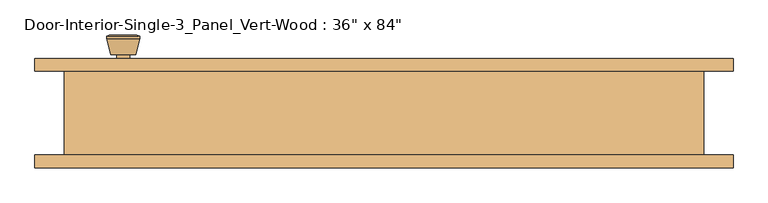
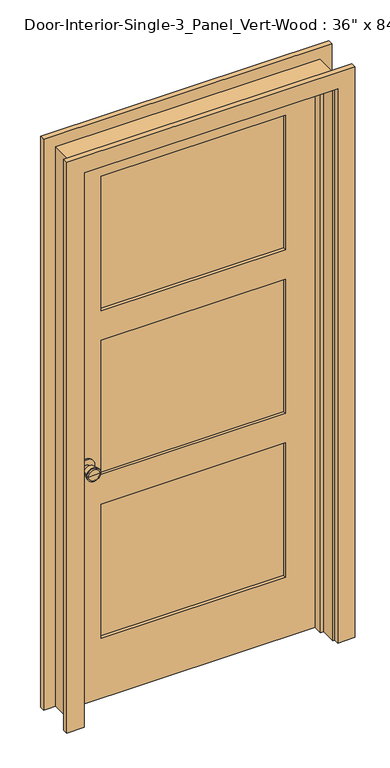
"""IFC4 building model written with IfcOpenShell, lengths in millimetres: door geometry."""

from ifc_helpers import new_model, si_unit, point, frame, frame_2d, origin, place, context, project, spatial, polyline, circle_curve, trimmed, segment, composite_curve, outline, extrude, faceted_brep, source, transform, mapped, element, save
from ifc_brep_helpers import plane_surface, cylinder_surface, revolved_surface, advanced_brep


def door_074fb280(model_context):
    return source(origin(), model_context, "Body", "SolidModel", [
        advanced_brep(
        [(-393.7, 19.4, 914.4), (-383.7, 19.4, 914.4), (-403.7, 19.4, 914.4), (-373.2241324, -29.6, 914.4), (-393.7, -29.6, 914.4), (-414.1758676, -29.6, 914.4), (-368.7, -27.7721319, 914.4), (-418.7, -27.7721319, 914.4), (-368.7, -24.3084537, 914.4), (-418.7, -24.3084537, 914.4), (-375.063764, 0.4, 914.4), (-412.336236, 0.4, 914.4), (-383.7, 0.4, 914.4), (-403.7, 0.4, 914.4)],
        [
            (0, 1),
            (1, 2, circle_curve(frame((-393.7, 19.4, 914.4), z_axis=(0.0, 1.0, 0.0), x_axis=(-1.0, 0.0, 0.0)), 10.0)),
            (2, 0),
            (2, 1, circle_curve(frame((-393.7, 19.4, 914.4), z_axis=(0.0, 1.0, 0.0), x_axis=(-1.0, 0.0, 0.0)), 10.0)),
            (3, 4),
            (4, 5),
            (5, 3, circle_curve(frame((-393.7, -29.6, 914.4), z_axis=(0.0, -1.0, 0.0), x_axis=(-1.0, 0.0, 0.0)), 20.4758676)),
            (3, 5, circle_curve(frame((-393.7, -29.6, 914.4), z_axis=(0.0, -1.0, 0.0), x_axis=(-1.0, 0.0, 0.0)), 20.4758676)),
            (6, 3),
            (5, 7),
            (7, 6, circle_curve(frame((-393.7, -27.7721319, 914.4), z_axis=(0.0, -1.0, 0.0), x_axis=(-1.0, 0.0, 0.0)), 25.0)),
            (6, 7, circle_curve(frame((-393.7, -27.7721319, 914.4), z_axis=(0.0, -1.0, 0.0), x_axis=(-1.0, 0.0, 0.0)), 25.0)),
            (8, 6),
            (7, 9),
            (9, 8, circle_curve(frame((-393.7, -24.3084537, 914.4), z_axis=(0.0, -1.0, 0.0), x_axis=(-1.0, 0.0, 0.0)), 25.0)),
            (8, 9, circle_curve(frame((-393.7, -24.3084537, 914.4), z_axis=(0.0, -1.0, 0.0), x_axis=(-1.0, 0.0, 0.0)), 25.0)),
            (10, 8),
            (9, 11),
            (11, 10, circle_curve(frame((-393.7, 0.4, 914.4), z_axis=(0.0, -1.0, 0.0), x_axis=(-1.0, 0.0, 0.0)), 18.636236)),
            (10, 11, circle_curve(frame((-393.7, 0.4, 914.4), z_axis=(0.0, -1.0, 0.0), x_axis=(-1.0, 0.0, 0.0)), 18.636236)),
            (12, 10),
            (11, 13),
            (13, 12, circle_curve(frame((-393.7, 0.4, 914.4), z_axis=(0.0, -1.0, 0.0), x_axis=(-1.0, 0.0, 0.0)), 10.0)),
            (12, 13, circle_curve(frame((-393.7, 0.4, 914.4), z_axis=(0.0, -1.0, 0.0), x_axis=(-1.0, 0.0, 0.0)), 10.0)),
            (1, 12),
            (13, 2),
        ],
        [
            plane_surface(frame((-393.7, 19.4, 914.4), z_axis=(0.0, 1.0, 0.0), x_axis=(-1.0, 0.0, 0.0))),
            plane_surface(frame((-393.7, -29.6, 914.4), z_axis=(0.0, -1.0, 0.0), x_axis=(-1.0, 0.0, 0.0))),
            revolved_surface(polyline([(-414.1758676, -29.6, 914.4), (-418.7, -27.7721319, 914.4)]), (-393.7, 19.4, 914.4), (0.0, 1.0, 0.0)),
            cylinder_surface(frame((-393.7, 19.4, 914.4), z_axis=(0.0, 1.0, 0.0), x_axis=(-1.0, 0.0, 0.0)), 25.0),
            revolved_surface(polyline([(-418.7, -24.3084537, 914.4), (-412.336236, 0.4, 914.4)]), (-393.7, 19.4, 914.4), (0.0, 1.0, 0.0)),
            plane_surface(frame((-393.7, 0.4, 914.4), z_axis=(0.0, 1.0, 0.0), x_axis=(-1.0, 0.0, 0.0))),
            cylinder_surface(frame((-393.7, 19.4, 914.4), z_axis=(0.0, 1.0, 0.0), x_axis=(-1.0, 0.0, 0.0)), 10.0),
        ],
        [
            (0, [[1, 2, 3]]),
            (0, [[-3, 4, -1]]),
            (1, [[5, 6, 7]]),
            (1, [[-6, -5, 8]]),
            (2, [[9, -7, 10, 11]]),
            (2, [[-10, -8, -9, 12]]),
            (3, [[13, -11, 14, 15]]),
            (3, [[-14, -12, -13, 16]]),
            (4, [[17, -15, 18, 19]]),
            (4, [[-18, -16, -17, 20]]),
            (5, [[21, -19, 22, 23]]),
            (5, [[-22, -20, -21, 24]]),
            (6, [[25, -23, 26, -2]]),
            (6, [[-26, -24, -25, -4]]),
        ],
    ),
        extrude(outline(composite_curve([segment(trimmed(circle_curve(frame_2d((914.4, -393.7)), 30.0), [point((914.4, -423.7))], [point((914.4, -363.7))], False, "CARTESIAN"), True, "CONTINUOUS"), segment(trimmed(circle_curve(frame_2d((914.4, -393.7)), 30.0), [point((914.4, -363.7))], [point((914.4, -423.7))], False, "CARTESIAN"), True, "CONTINUOUS")], self_intersect=False)), frame((0.0, 19.4, 0.0), z_axis=(0.0, 1.0, 0.0), x_axis=(0.0, 0.0, 1.0)), (0.0, 0.0, 1.0), 6.0),
        advanced_brep(
        [(-393.7, 66.325, 914.4), (-403.7, 66.325, 914.4), (-383.7, 66.325, 914.4), (-373.2241324, 115.325, 914.4), (-414.1758676, 115.325, 914.4), (-393.7, 115.325, 914.4), (-368.7, 113.4971319, 914.4), (-418.7, 113.4971319, 914.4), (-368.7, 110.0334537, 914.4), (-418.7, 110.0334537, 914.4), (-375.063764, 85.325, 914.4), (-412.336236, 85.325, 914.4), (-383.7, 85.325, 914.4), (-403.7, 85.325, 914.4)],
        [
            (0, 1),
            (1, 2, circle_curve(frame((-393.7, 66.325, 914.4), z_axis=(0.0, -1.0, 0.0), x_axis=(-1.0, 0.0, 0.0)), 10.0)),
            (2, 0),
            (2, 1, circle_curve(frame((-393.7, 66.325, 914.4), z_axis=(0.0, -1.0, 0.0), x_axis=(-1.0, 0.0, 0.0)), 10.0)),
            (3, 4, circle_curve(frame((-393.7, 115.325, 914.4), z_axis=(0.0, 1.0, 0.0), x_axis=(-1.0, 0.0, 0.0)), 20.4758676)),
            (4, 5),
            (5, 3),
            (4, 3, circle_curve(frame((-393.7, 115.325, 914.4), z_axis=(0.0, 1.0, 0.0), x_axis=(-1.0, 0.0, 0.0)), 20.4758676)),
            (6, 7, circle_curve(frame((-393.7, 113.4971319, 914.4), z_axis=(0.0, 1.0, 0.0), x_axis=(-1.0, 0.0, 0.0)), 25.0)),
            (7, 4),
            (3, 6),
            (7, 6, circle_curve(frame((-393.7, 113.4971319, 914.4), z_axis=(0.0, 1.0, 0.0), x_axis=(-1.0, 0.0, 0.0)), 25.0)),
            (8, 9, circle_curve(frame((-393.7, 110.0334537, 914.4), z_axis=(0.0, 1.0, 0.0), x_axis=(-1.0, 0.0, 0.0)), 25.0)),
            (9, 7),
            (6, 8),
            (9, 8, circle_curve(frame((-393.7, 110.0334537, 914.4), z_axis=(0.0, 1.0, 0.0), x_axis=(-1.0, 0.0, 0.0)), 25.0)),
            (10, 11, circle_curve(frame((-393.7, 85.325, 914.4), z_axis=(0.0, 1.0, 0.0), x_axis=(-1.0, 0.0, 0.0)), 18.636236)),
            (11, 9),
            (8, 10),
            (11, 10, circle_curve(frame((-393.7, 85.325, 914.4), z_axis=(0.0, 1.0, 0.0), x_axis=(-1.0, 0.0, 0.0)), 18.636236)),
            (12, 13, circle_curve(frame((-393.7, 85.325, 914.4), z_axis=(0.0, 1.0, 0.0), x_axis=(-1.0, 0.0, 0.0)), 10.0)),
            (13, 11),
            (10, 12),
            (13, 12, circle_curve(frame((-393.7, 85.325, 914.4), z_axis=(0.0, 1.0, 0.0), x_axis=(-1.0, 0.0, 0.0)), 10.0)),
            (1, 13),
            (12, 2),
        ],
        [
            plane_surface(frame((-393.7, 66.325, 914.4), z_axis=(0.0, -1.0, 0.0), x_axis=(-1.0, 0.0, 0.0))),
            plane_surface(frame((-393.7, 115.325, 914.4), z_axis=(0.0, 1.0, 0.0), x_axis=(-1.0, 0.0, 0.0))),
            revolved_surface(polyline([(-414.1758676, 115.325, 914.4), (-418.7, 113.4971319, 914.4)]), (-393.7, 66.325, 914.4), (0.0, -1.0, 0.0)),
            cylinder_surface(frame((-393.7, 66.325, 914.4), z_axis=(0.0, -1.0, 0.0), x_axis=(-1.0, 0.0, 0.0)), 25.0),
            revolved_surface(polyline([(-418.7, 110.0334537, 914.4), (-412.336236, 85.325, 914.4)]), (-393.7, 66.325, 914.4), (0.0, -1.0, 0.0)),
            plane_surface(frame((-393.7, 85.325, 914.4), z_axis=(0.0, -1.0, 0.0), x_axis=(-1.0, 0.0, 0.0))),
            cylinder_surface(frame((-393.7, 66.325, 914.4), z_axis=(0.0, -1.0, 0.0), x_axis=(-1.0, 0.0, 0.0)), 10.0),
        ],
        [
            (0, [[1, 2, 3]]),
            (0, [[-3, 4, -1]]),
            (1, [[5, 6, 7]]),
            (1, [[8, -7, -6]]),
            (2, [[9, 10, -5, 11]]),
            (2, [[12, -11, -8, -10]]),
            (3, [[13, 14, -9, 15]]),
            (3, [[16, -15, -12, -14]]),
            (4, [[17, 18, -13, 19]]),
            (4, [[20, -19, -16, -18]]),
            (5, [[21, 22, -17, 23]]),
            (5, [[24, -23, -20, -22]]),
            (6, [[-2, 25, -21, 26]]),
            (6, [[-4, -26, -24, -25]]),
        ],
    ),
        extrude(outline(composite_curve([segment(trimmed(circle_curve(frame_2d((914.4, -393.7)), 30.0), [point((914.4, -423.7))], [point((914.4, -363.7))], False, "CARTESIAN"), True, "CONTINUOUS"), segment(trimmed(circle_curve(frame_2d((914.4, -393.7)), 30.0), [point((914.4, -363.7))], [point((914.4, -423.7))], False, "CARTESIAN"), True, "CONTINUOUS")], self_intersect=False)), frame((0.0, 60.325, 0.0), z_axis=(0.0, 1.0, 0.0), x_axis=(0.0, 0.0, 1.0)), (0.0, 0.0, 1.0), 6.0),
        extrude(outline(polyline([(336.55, 37.0416667), (-336.55, 37.0416667), (-336.55, 48.6833333), (336.55, 48.6833333), (336.55, 37.0416667)])), frame((0.0, 0.0, 1496.4833333), z_axis=(0.0, 0.0, 1.0), x_axis=(1.0, 0.0, 0.0)), (0.0, 0.0, 1.0), 518.0541667),
        extrude(outline(polyline([(336.55, 37.0416667), (-336.55, 37.0416667), (-336.55, 48.6833333), (336.55, 48.6833333), (336.55, 37.0416667)])), frame((0.0, 0.0, 231.775), z_axis=(0.0, 0.0, 1.0), x_axis=(1.0, 0.0, 0.0)), (0.0, 0.0, 1.0), 518.0541667),
        extrude(outline(polyline([(336.55, 37.0416667), (-336.55, 37.0416667), (-336.55, 48.6833333), (336.55, 48.6833333), (336.55, 37.0416667)])), frame((0.0, 0.0, 864.1291667), z_axis=(0.0, 0.0, 1.0), x_axis=(1.0, 0.0, 0.0)), (0.0, 0.0, 1.0), 518.0541667),
        extrude(outline(polyline([(2133.6, -457.2), (0.0, -457.2), (0.0, 457.2), (2133.6, 457.2), (2133.6, -457.2)]), holes=[polyline([(2014.5375, -336.55), (2014.5375, 336.55), (1496.4833333, 336.55), (1496.4833333, -336.55), (2014.5375, -336.55)]), polyline([(749.8291667, -336.55), (749.8291667, 336.55), (231.775, 336.55), (231.775, -336.55), (749.8291667, -336.55)]), polyline([(1382.1833333, -336.55), (1382.1833333, 336.55), (864.1291667, 336.55), (864.1291667, -336.55), (1382.1833333, -336.55)])]), frame((0.0, 25.4, 0.0), z_axis=(0.0, 1.0, 0.0), x_axis=(0.0, 0.0, 1.0)), (0.0, 0.0, 1.0), 34.925),
        faceted_brep([(482.6, 60.325, 0.0), (482.6, -66.675, 0.0), (457.2, -66.675, 0.0), (457.2, -9.525, 0.0), (444.5, -9.525, 0.0), (444.5, 25.4, 0.0), (457.2, 25.4, 0.0), (457.2, 60.325, 0.0), (482.6, 60.325, 2159.0), (482.6, -66.675, 2159.0), (-482.6, -66.675, 2159.0), (-482.6, -66.675, 0.0), (-457.2, -66.675, 0.0), (-457.2, -66.675, 2133.6), (457.2, -66.675, 2133.6), (457.2, -9.525, 2133.6), (-457.2, -9.525, 2133.6), (-457.2, -9.525, 0.0), (-444.5, -9.525, 0.0), (-444.5, -9.525, 2120.9), (444.5, -9.525, 2120.9), (444.5, 25.4, 2120.9), (-444.5, 25.4, 2120.9), (-444.5, 25.4, 0.0), (-457.2, 25.4, 0.0), (-457.2, 25.4, 2133.6), (457.2, 25.4, 2133.6), (457.2, 60.325, 2133.6), (-457.2, 60.325, 2133.6), (-457.2, 60.325, 0.0), (-482.6, 60.325, 0.0), (-482.6, 60.325, 2159.0)], [[[0, 1, 2, 3, 4, 5, 6, 7]], [[1, 0, 8, 9]], [[2, 1, 9, 10, 11, 12, 13, 14]], [[3, 2, 14, 15]], [[4, 3, 15, 16, 17, 18, 19, 20]], [[5, 4, 20, 21]], [[6, 5, 21, 22, 23, 24, 25, 26]], [[7, 6, 26, 27]], [[0, 7, 27, 28, 29, 30, 31, 8]], [[9, 8, 31, 10]], [[15, 14, 13, 16]], [[21, 20, 19, 22]], [[27, 26, 25, 28]], [[30, 29, 24, 23, 18, 17, 12, 11]], [[10, 31, 30, 11]], [[16, 13, 12, 17]], [[22, 19, 18, 23]], [[28, 25, 24, 29]]]),
        extrude(outline(polyline([(0.0, 463.55), (0.0, 527.05), (2203.45, 527.05), (2203.45, -527.05), (0.0, -527.05), (0.0, -463.55), (2139.95, -463.55), (2139.95, 463.55), (0.0, 463.55)])), frame((0.0, -85.725, 0.0), z_axis=(0.0, 1.0, 0.0), x_axis=(0.0, 0.0, 1.0)), (0.0, 0.0, 1.0), 19.05),
        extrude(outline(polyline([(0.0, 463.55), (0.0, 527.05), (2203.45, 527.05), (2203.45, -527.05), (0.0, -527.05), (0.0, -463.55), (2139.95, -463.55), (2139.95, 463.55), (0.0, 463.55)])), frame((0.0, 60.325, 0.0), z_axis=(0.0, 1.0, 0.0), x_axis=(0.0, 0.0, 1.0)), (0.0, 0.0, 1.0), 19.05),
    ])


if __name__ == "__main__":
    model = new_model("IFC4")
    model_context = context("Model", 3, world=origin())
    ifc_project = project(units=[si_unit("LENGTHUNIT", "METRE", prefix="MILLI")], contexts=[model_context])
    site = spatial("IfcSite", under=ifc_project)
    building = spatial("IfcBuilding", under=site)
    placement = place(None, origin())
    door_shape = door_074fb280(model_context)
    element("IfcDoor", 1, ObjectType="Door-Interior-Single-3_Panel_Vert-Wood : 36\" x 84\"", at=placement, inside=building, context=model_context, shape_type="MappedRepresentation", body=[
        mapped(door_shape, transform((0.0, 0.0, 0.0), x_axis=(1.0, 0.0, 0.0), y_axis=(0.0, 1.0, 0.0), z_axis=(0.0, 0.0, 1.0))),
    ])
    save(model, "model.ifc")

# Revit data of these elements
# Project information
#   Project Issue Date = "Issue Date"
#   Project Status = "Project Status"
#   Client Name = "Owner"
#   Project Address = "Enter address here"
#   Project Name = "Project Name"
#   Project Number = "Project Number"
# Type "Door-Interior-Single-3_Panel_Vert-Wood : 36\" x 84\""
#   Type Mark = "10"
#   Assembly Code = "C1020300"
#   Analytic Construction = "Wooden"
#   Top Rail = 0' - 4 11/16"
#   Thickness = 0' - 1 3/8"
#   Thermal Resistance (R) = 2.5876 (h·ft²·°F)/BTU
#   Swing Angle [instance default] = 90.00°
#   Stiles = 0' - 4 3/4"
#   Rough Width = 3' - 2"
#   Rough Height = 7' - 1"
#   Intermediate Rail = 0' - 4 1/2"
#   Height = 7' - 0"
#   Width = 3' - 0"
#   Heat Transfer Coefficient (U) = 0.3865 BTU/(h·ft²·°F)
#   Bottom Rail = 0' - 9 1/8"
#   Trim Material = Cherry
#   Panel Material = Cherry
#   Frame Material = Cherry
#   Door Handle Material = Aluminum
#   Visual Light Transmittance = 0
#   Solar Heat Gain Coefficient = 0
#   Wall Closure = (empty or 0)
#   Function = (empty or 0)
# Element 1 (IfcDoor, "Door-Interior-Single-3_Panel_Vert-Wood : 36\" x 84\"")
#   Materials on its faces: "Cherry", "Aluminum"
# Materials
#   "Cherry": class "Wood", colour RGB 226 177 128, transparency 0, Description = "Prunus Serotina", Cost = 0
#   "Aluminum": class "Metal", colour RGB 247 247 247, transparency 0, Description = "Aluminum 6061", Cost = 0
